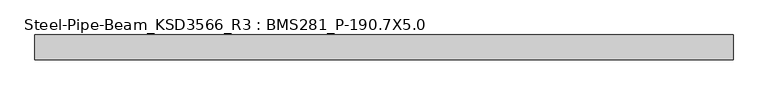
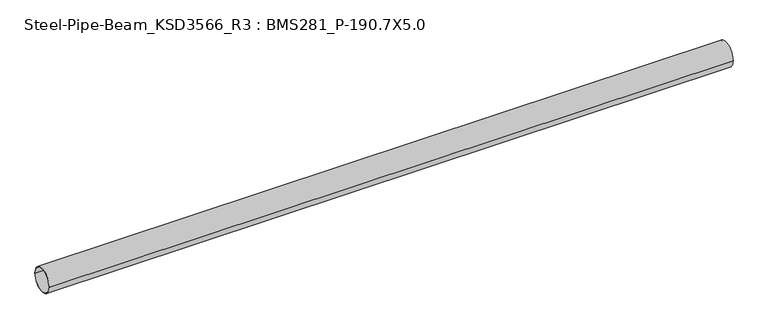
"""IFC4 building model written with IfcOpenShell, lengths in millimetres: member geometry, Steel-Pipe-Beam_KSD3566_R3 : BMS281_P-190.7X5.0."""

import ifcopenshell
import ifcopenshell.guid

model = None  # the IFC model being written
_history = None  # IfcOwnerHistory: only IFC2X3 demands one
_inside = {}  # id of a spatial element -> (the spatial element, [elements in it])
_under = {}  # id of a project, library or spatial element -> (it, [spatial elements below it])
_declared = {}  # id of a project -> (the project, [libraries it declares])
_typed = {}  # id of a type object -> (the type object, [elements of that type])
_made_of = {}  # id of a material, layer set ... -> (it, [elements and type objects made of it])


def new_model(schema):
    """Start an empty IFC model of exactly this schema.

    Asked for "IFC4X3", IfcOpenShell would pick the latest addendum, in which some entities
    have other attributes; the version numbers below select the first issue.
    IFC2X3 requires an IfcOwnerHistory on every rooted entity: one is made here for all.
    """
    global model, _history
    if schema == "IFC4X3":
        model = ifcopenshell.file(schema_version=(4, 3, 0, 0))
    else:
        model = ifcopenshell.file(schema=schema)
    _inside.clear()
    _under.clear()
    _declared.clear()
    _typed.clear()
    _made_of.clear()
    _history = None
    if model.schema == "IFC2X3":
        org = make("IfcOrganization", Name="unknown")
        user = make(
            "IfcPersonAndOrganization",
            ThePerson=make("IfcPerson", FamilyName="unknown"),
            TheOrganization=org,
        )
        app = make(
            "IfcApplication",
            ApplicationDeveloper=org,
            Version="unknown",
            ApplicationFullName="unknown",
            ApplicationIdentifier="unknown",
        )
        _history = make(
            "IfcOwnerHistory",
            OwningUser=user,
            OwningApplication=app,
            ChangeAction="ADDED",
            CreationDate=0,
        )
    return model


def make(cls, **values):
    """One entity of the class cls with the attributes given. An attribute that is None is left unset."""
    return model.create_entity(
        cls, **{name: value for name, value in values.items() if value is not None}
    )


def rooted(cls, **values):
    """An entity with a GlobalId (a new one), such as an element, a storey or a relation."""
    return make(cls, GlobalId=ifcopenshell.guid.new(), OwnerHistory=_history, **values)


def si_unit(unit_type, name, prefix=None):
    """IfcSIUnit, for example si_unit("LENGTHUNIT", "METRE", prefix="MILLI")."""
    return make("IfcSIUnit", UnitType=unit_type, Prefix=prefix, Name=name)


def assignment(units):
    """IfcUnitAssignment: the units of a project."""
    return None if units is None else make("IfcUnitAssignment", Units=units)


def point(xyz):
    """IfcCartesianPoint."""
    return None if xyz is None else make("IfcCartesianPoint", Coordinates=xyz)


def direction(xyz):
    """IfcDirection."""
    return None if xyz is None else make("IfcDirection", DirectionRatios=xyz)


def frame(location, z_axis=None, x_axis=None):
    """IfcAxis2Placement3D, a coordinate frame: its origin and axes. An axis left out is left unset."""
    return make(
        "IfcAxis2Placement3D",
        Location=point(location),
        Axis=direction(z_axis),
        RefDirection=direction(x_axis),
    )


def frame_2d(location, x_axis=None):
    """IfcAxis2Placement2D, a coordinate frame in the plane: its origin and x axis."""
    return make(
        "IfcAxis2Placement2D", Location=point(location), RefDirection=direction(x_axis)
    )


def origin():
    """The frame at (0, 0, 0) with its axes left unset."""
    return frame((0.0, 0.0, 0.0))


def origin_2d():
    """The frame at (0, 0) in the plane with its x axis left unset."""
    return frame_2d((0.0, 0.0))


def place(relative_to, where):
    """IfcLocalPlacement: puts the frame where relative to a parent placement (None: the world)."""
    return make(
        "IfcLocalPlacement", PlacementRelTo=relative_to, RelativePlacement=where
    )


def context(
    kind, dimensions, precision=None, world=None, true_north=None, identifier=None
):
    """IfcGeometricRepresentationContext, for example the 3D "Model" context."""
    return make(
        "IfcGeometricRepresentationContext",
        ContextIdentifier=identifier,
        ContextType=kind,
        CoordinateSpaceDimension=dimensions,
        Precision=precision,
        WorldCoordinateSystem=world,
        TrueNorth=true_north,
    )


def project(units=None, contexts=None):
    """IfcProject with its units and contexts."""
    return rooted(
        "IfcProject",
        Name="project",
        RepresentationContexts=contexts,
        UnitsInContext=assignment(units),
    )


def spatial(cls, under=None, at=None, **own):
    """A site, building, storey or space (cls), placed at a placement, below another one or the project."""
    s = rooted(cls, ObjectPlacement=at, **own)
    if under is not None:
        _under.setdefault(under.id(), (under, []))[1].append(s)
    return s


def circle_curve(where, radius):
    """IfcCircle in the frame where."""
    return make("IfcCircle", Position=where, Radius=radius)


def trimmed(basis, trim1, trim2, sense, master):
    """IfcTrimmedCurve: the piece of a basis curve between two trims."""
    return make(
        "IfcTrimmedCurve",
        BasisCurve=basis,
        Trim1=trim1,
        Trim2=trim2,
        SenseAgreement=sense,
        MasterRepresentation=master,
    )


def segment(curve, same_sense, transition):
    """IfcCompositeCurveSegment."""
    return make(
        "IfcCompositeCurveSegment",
        Transition=transition,
        SameSense=same_sense,
        ParentCurve=curve,
    )


def composite_curve(segments, self_intersect=None):
    """IfcCompositeCurve: segments joined end to end."""
    return make("IfcCompositeCurve", Segments=segments, SelfIntersect=self_intersect)


def outline(outer, holes=None, kind="AREA"):
    """IfcArbitraryClosedProfileDef: a profile drawn as a closed curve; with holes, ...WithVoids."""
    if holes is None:
        return make("IfcArbitraryClosedProfileDef", ProfileType=kind, OuterCurve=outer)
    return make(
        "IfcArbitraryProfileDefWithVoids",
        ProfileType=kind,
        OuterCurve=outer,
        InnerCurves=holes,
    )


def extrude(swept, where, along, depth):
    """IfcExtrudedAreaSolid: the profile swept, set in the frame where, extruded along a direction by depth."""
    return make(
        "IfcExtrudedAreaSolid",
        SweptArea=swept,
        Position=where,
        ExtrudedDirection=direction(along),
        Depth=depth,
    )


def shape(context_of_items, identifier, shape_type, items):
    """IfcShapeRepresentation: the items that make up one representation, for example the "Body"."""
    return make(
        "IfcShapeRepresentation",
        ContextOfItems=context_of_items,
        RepresentationIdentifier=identifier,
        RepresentationType=shape_type,
        Items=items,
    )


def source(mapping_origin, context_of_items, identifier, shape_type, items):
    """IfcRepresentationMap: a shape defined once, which mapped items show again and again."""
    return make(
        "IfcRepresentationMap",
        MappingOrigin=mapping_origin,
        MappedRepresentation=shape(context_of_items, identifier, shape_type, items),
    )


def transform(
    local_origin,
    x_axis=None,
    y_axis=None,
    z_axis=None,
    scale=None,
    scale2=None,
    scale3=None,
    uniform=True,
):
    """IfcCartesianTransformationOperator3D, or its non-uniform kind. x_axis, y_axis, z_axis: its Axis1, 2, 3."""
    if uniform:
        return make(
            "IfcCartesianTransformationOperator3D",
            Axis1=direction(x_axis),
            Axis2=direction(y_axis),
            LocalOrigin=point(local_origin),
            Scale=scale,
            Axis3=direction(z_axis),
        )
    return make(
        "IfcCartesianTransformationOperator3DnonUniform",
        Axis1=direction(x_axis),
        Axis2=direction(y_axis),
        LocalOrigin=point(local_origin),
        Scale=scale,
        Axis3=direction(z_axis),
        Scale2=scale2,
        Scale3=scale3,
    )


def mapped(mapping_source, mapping_target):
    """IfcMappedItem: shows the shape of a source again, moved by a transform."""
    return make(
        "IfcMappedItem", MappingSource=mapping_source, MappingTarget=mapping_target
    )


def made_of(thing, what):
    """Note that an element or type object is made of a material, layer set ...; save() writes the relation."""
    if what is not None:
        _made_of.setdefault(what.id(), (what, []))[1].append(thing)
    return thing


def element(
    cls,
    number,
    at=None,
    inside=None,
    cuts=None,
    type_object=None,
    material=None,
    context=None,
    identifier="Body",
    shape_type=None,
    held_by="IfcProductDefinitionShape",
    body=None,
    shapes=None,
    **own,
):
    """One element of the class cls, such as IfcWall. Its Tag is "e" and its number.

    at: its placement. inside: the storey or other place that contains it. cuts: it is an
    opening in that element (IfcRelVoidsElement). A single representation is given by context,
    identifier, shape_type and body (its items); several are given by shapes. held_by: the class
    of the entity that holds the representations. save() writes the other relations.
    """
    e = rooted(cls, Tag="e%d" % number, ObjectPlacement=at, **own)
    if body is not None:
        shapes = [shape(context, identifier, shape_type, body)]
    if shapes is not None:
        e.Representation = make(held_by, Representations=shapes)
    if inside is not None:
        _inside.setdefault(inside.id(), (inside, []))[1].append(e)
    if cuts is not None:
        rooted(
            "IfcRelVoidsElement", RelatingBuildingElement=cuts, RelatedOpeningElement=e
        )
    if type_object is not None:
        _typed.setdefault(type_object.id(), (type_object, []))[1].append(e)
    return made_of(e, material)


def aggregate(whole, parts):
    """IfcRelAggregates: a whole, such as a stair, and the parts it consists of."""
    return rooted("IfcRelAggregates", RelatingObject=whole, RelatedObjects=parts)


def save(model, path):
    """Write the relations noted so far, then the file.

    IfcRelAggregates (storeys below a building ...), IfcRelContainedInSpatialStructure (elements
    in a storey), IfcRelDefinesByType, IfcRelAssociatesMaterial and IfcRelDeclares: one each for
    every whole, place, type object, material and project.
    """
    for whole, parts in _under.values():
        aggregate(whole, parts)
    for where, things in _inside.values():
        rooted(
            "IfcRelContainedInSpatialStructure",
            RelatedElements=things,
            RelatingStructure=where,
        )
    for kind, things in _typed.values():
        rooted("IfcRelDefinesByType", RelatedObjects=things, RelatingType=kind)
    for what, things in _made_of.values():
        rooted("IfcRelAssociatesMaterial", RelatedObjects=things, RelatingMaterial=what)
    for by, libraries in _declared.values():
        rooted("IfcRelDeclares", RelatingContext=by, RelatedDefinitions=libraries)
    model.write(path)


def steel_pipe_beam_ksd3566_r3_bms281_p_190_7x5_0_12fd126f(model_context):
    return source(origin(), model_context, "Body", "SweptSolid", [
        extrude(outline(composite_curve([segment(trimmed(circle_curve(origin_2d(), 95.35), [point((-95.35, 0.0))], [point((95.35, 0.0))], False, "CARTESIAN"), True, "CONTINUOUS"), segment(trimmed(circle_curve(origin_2d(), 95.35), [point((95.35, 0.0))], [point((-95.35, 0.0))], False, "CARTESIAN"), True, "CONTINUOUS")], self_intersect=False), holes=[composite_curve([segment(trimmed(circle_curve(origin_2d(), 90.35), [point((90.35, 0.0))], [point((-90.35, 0.0))], True, "CARTESIAN"), True, "CONTINUOUS"), segment(trimmed(circle_curve(origin_2d(), 90.35), [point((-90.35, 0.0))], [point((90.35, 0.0))], True, "CARTESIAN"), True, "CONTINUOUS")], self_intersect=False)]), frame((-2577.1305565, 0.0, 0.0), z_axis=(1.0, 0.0, 0.0), x_axis=(0.0, 1.0, 0.0)), (0.0, 0.0, 1.0), 5312.4906205),
    ])


if __name__ == "__main__":
    model = new_model("IFC4")
    model_context = context("Model", 3, world=origin())
    ifc_project = project(units=[si_unit("LENGTHUNIT", "METRE", prefix="MILLI")], contexts=[model_context])
    site = spatial("IfcSite", under=ifc_project)
    building = spatial("IfcBuilding", under=site)
    placement = place(None, origin())
    steel_pipe_beam_ksd3566_r3_bms281_p_190_7x5_0_shape = steel_pipe_beam_ksd3566_r3_bms281_p_190_7x5_0_12fd126f(model_context)
    element("IfcMember", 1, ObjectType="Steel-Pipe-Beam_KSD3566_R3 : BMS281_P-190.7X5.0", at=placement, inside=building, context=model_context, shape_type="MappedRepresentation", body=[
        mapped(steel_pipe_beam_ksd3566_r3_bms281_p_190_7x5_0_shape, transform((0.0, 0.0, 0.0), x_axis=(1.0, 0.0, 0.0), y_axis=(0.0, 1.0, 0.0), z_axis=(0.0, 0.0, 1.0))),
    ])
    save(model, "model.ifc")

# Revit data of these elements
# Type "Steel-Pipe-Beam_KSD3566_R3 : BMS281_P-190.7X5.0"
#   Keynote = "P-190.7X5.0"
#   SteelWeight = "Light"
#   t = 0.0050 m
#   Surface Area = 0.599102 m²/m
#   Section Area = 29.1697 cm²
#   Mass per Unit Length = 22.8982 kg/m
#   Length [instance default] = 1.5000 m
#   D = 0.1907 m
#   hec_material4 [instance default] = none
#   hec_material3 [instance default] = none
#   hec_material2 [instance default] = none
#   hec_material1 [instance default] = none
#   Structural Material [instance default] = Steel, 45-345
#   Assembly Code = ""
# Element 1 (IfcMember, "Steel-Pipe-Beam_KSD3566_R3 : BMS281_P-190.7X5.0")
#   Structural Material = none
# Materials
#   "Steel, 45-345": class "Metal", colour RGB 189 187 185, transparency 0, Description = "Steel 345 MPa", Cost = 0
